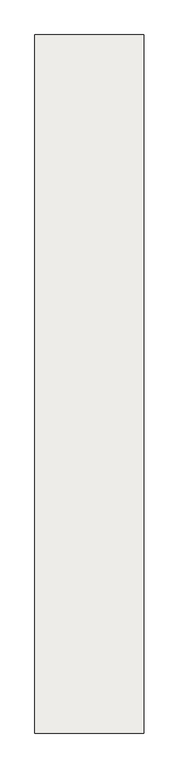
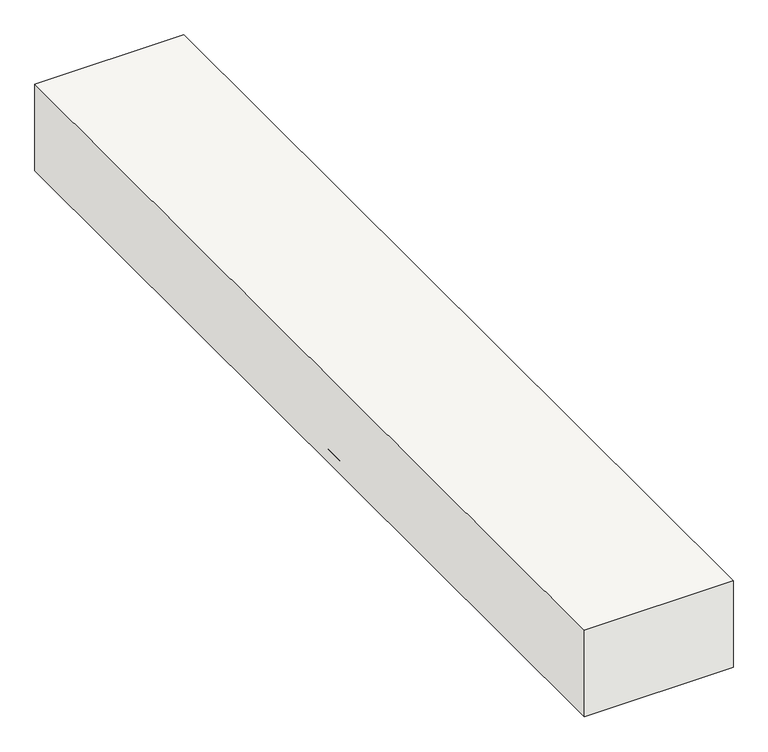
"""IFC4 building model written with IfcOpenShell, lengths in millimetres: slab geometry, Pano 16 (16 cm)."""

import ifcopenshell
import ifcopenshell.guid

model = None  # the IFC model being written
_history = None  # IfcOwnerHistory: only IFC2X3 demands one
_inside = {}  # id of a spatial element -> (the spatial element, [elements in it])
_under = {}  # id of a project, library or spatial element -> (it, [spatial elements below it])
_declared = {}  # id of a project -> (the project, [libraries it declares])
_typed = {}  # id of a type object -> (the type object, [elements of that type])
_made_of = {}  # id of a material, layer set ... -> (it, [elements and type objects made of it])


def new_model(schema):
    """Start an empty IFC model of exactly this schema.

    Asked for "IFC4X3", IfcOpenShell would pick the latest addendum, in which some entities
    have other attributes; the version numbers below select the first issue.
    IFC2X3 requires an IfcOwnerHistory on every rooted entity: one is made here for all.
    """
    global model, _history
    if schema == "IFC4X3":
        model = ifcopenshell.file(schema_version=(4, 3, 0, 0))
    else:
        model = ifcopenshell.file(schema=schema)
    _inside.clear()
    _under.clear()
    _declared.clear()
    _typed.clear()
    _made_of.clear()
    _history = None
    if model.schema == "IFC2X3":
        org = make("IfcOrganization", Name="unknown")
        user = make(
            "IfcPersonAndOrganization",
            ThePerson=make("IfcPerson", FamilyName="unknown"),
            TheOrganization=org,
        )
        app = make(
            "IfcApplication",
            ApplicationDeveloper=org,
            Version="unknown",
            ApplicationFullName="unknown",
            ApplicationIdentifier="unknown",
        )
        _history = make(
            "IfcOwnerHistory",
            OwningUser=user,
            OwningApplication=app,
            ChangeAction="ADDED",
            CreationDate=0,
        )
    return model


def make(cls, **values):
    """One entity of the class cls with the attributes given. An attribute that is None is left unset."""
    return model.create_entity(
        cls, **{name: value for name, value in values.items() if value is not None}
    )


def rooted(cls, **values):
    """An entity with a GlobalId (a new one), such as an element, a storey or a relation."""
    return make(cls, GlobalId=ifcopenshell.guid.new(), OwnerHistory=_history, **values)


def si_unit(unit_type, name, prefix=None):
    """IfcSIUnit, for example si_unit("LENGTHUNIT", "METRE", prefix="MILLI")."""
    return make("IfcSIUnit", UnitType=unit_type, Prefix=prefix, Name=name)


def assignment(units):
    """IfcUnitAssignment: the units of a project."""
    return None if units is None else make("IfcUnitAssignment", Units=units)


def point(xyz):
    """IfcCartesianPoint."""
    return None if xyz is None else make("IfcCartesianPoint", Coordinates=xyz)


def direction(xyz):
    """IfcDirection."""
    return None if xyz is None else make("IfcDirection", DirectionRatios=xyz)


def frame(location, z_axis=None, x_axis=None):
    """IfcAxis2Placement3D, a coordinate frame: its origin and axes. An axis left out is left unset."""
    return make(
        "IfcAxis2Placement3D",
        Location=point(location),
        Axis=direction(z_axis),
        RefDirection=direction(x_axis),
    )


def origin():
    """The frame at (0, 0, 0) with its axes left unset."""
    return frame((0.0, 0.0, 0.0))


def origin_with_axes():
    """The frame at (0, 0, 0) with the z axis (0, 0, 1) and the x axis (1, 0, 0) written out."""
    return frame((0.0, 0.0, 0.0), z_axis=(0.0, 0.0, 1.0), x_axis=(1.0, 0.0, 0.0))


def place(relative_to, where):
    """IfcLocalPlacement: puts the frame where relative to a parent placement (None: the world)."""
    return make(
        "IfcLocalPlacement", PlacementRelTo=relative_to, RelativePlacement=where
    )


def context(
    kind, dimensions, precision=None, world=None, true_north=None, identifier=None
):
    """IfcGeometricRepresentationContext, for example the 3D "Model" context."""
    return make(
        "IfcGeometricRepresentationContext",
        ContextIdentifier=identifier,
        ContextType=kind,
        CoordinateSpaceDimension=dimensions,
        Precision=precision,
        WorldCoordinateSystem=world,
        TrueNorth=true_north,
    )


def project(units=None, contexts=None):
    """IfcProject with its units and contexts."""
    return rooted(
        "IfcProject",
        Name="project",
        RepresentationContexts=contexts,
        UnitsInContext=assignment(units),
    )


def spatial(cls, under=None, at=None, **own):
    """A site, building, storey or space (cls), placed at a placement, below another one or the project."""
    s = rooted(cls, ObjectPlacement=at, **own)
    if under is not None:
        _under.setdefault(under.id(), (under, []))[1].append(s)
    return s


def polyline(points):
    """IfcPolyline through the points."""
    return make("IfcPolyline", Points=[point(p) for p in points])


def outline(outer, holes=None, kind="AREA"):
    """IfcArbitraryClosedProfileDef: a profile drawn as a closed curve; with holes, ...WithVoids."""
    if holes is None:
        return make("IfcArbitraryClosedProfileDef", ProfileType=kind, OuterCurve=outer)
    return make(
        "IfcArbitraryProfileDefWithVoids",
        ProfileType=kind,
        OuterCurve=outer,
        InnerCurves=holes,
    )


def extrude(swept, where, along, depth):
    """IfcExtrudedAreaSolid: the profile swept, set in the frame where, extruded along a direction by depth."""
    return make(
        "IfcExtrudedAreaSolid",
        SweptArea=swept,
        Position=where,
        ExtrudedDirection=direction(along),
        Depth=depth,
    )


def shape(context_of_items, identifier, shape_type, items):
    """IfcShapeRepresentation: the items that make up one representation, for example the "Body"."""
    return make(
        "IfcShapeRepresentation",
        ContextOfItems=context_of_items,
        RepresentationIdentifier=identifier,
        RepresentationType=shape_type,
        Items=items,
    )


def source(mapping_origin, context_of_items, identifier, shape_type, items):
    """IfcRepresentationMap: a shape defined once, which mapped items show again and again."""
    return make(
        "IfcRepresentationMap",
        MappingOrigin=mapping_origin,
        MappedRepresentation=shape(context_of_items, identifier, shape_type, items),
    )


def transform(
    local_origin,
    x_axis=None,
    y_axis=None,
    z_axis=None,
    scale=None,
    scale2=None,
    scale3=None,
    uniform=True,
):
    """IfcCartesianTransformationOperator3D, or its non-uniform kind. x_axis, y_axis, z_axis: its Axis1, 2, 3."""
    if uniform:
        return make(
            "IfcCartesianTransformationOperator3D",
            Axis1=direction(x_axis),
            Axis2=direction(y_axis),
            LocalOrigin=point(local_origin),
            Scale=scale,
            Axis3=direction(z_axis),
        )
    return make(
        "IfcCartesianTransformationOperator3DnonUniform",
        Axis1=direction(x_axis),
        Axis2=direction(y_axis),
        LocalOrigin=point(local_origin),
        Scale=scale,
        Axis3=direction(z_axis),
        Scale2=scale2,
        Scale3=scale3,
    )


def mapped(mapping_source, mapping_target):
    """IfcMappedItem: shows the shape of a source again, moved by a transform."""
    return make(
        "IfcMappedItem", MappingSource=mapping_source, MappingTarget=mapping_target
    )


def made_of(thing, what):
    """Note that an element or type object is made of a material, layer set ...; save() writes the relation."""
    if what is not None:
        _made_of.setdefault(what.id(), (what, []))[1].append(thing)
    return thing


def element(
    cls,
    number,
    at=None,
    inside=None,
    cuts=None,
    type_object=None,
    material=None,
    context=None,
    identifier="Body",
    shape_type=None,
    held_by="IfcProductDefinitionShape",
    body=None,
    shapes=None,
    **own,
):
    """One element of the class cls, such as IfcWall. Its Tag is "e" and its number.

    at: its placement. inside: the storey or other place that contains it. cuts: it is an
    opening in that element (IfcRelVoidsElement). A single representation is given by context,
    identifier, shape_type and body (its items); several are given by shapes. held_by: the class
    of the entity that holds the representations. save() writes the other relations.
    """
    e = rooted(cls, Tag="e%d" % number, ObjectPlacement=at, **own)
    if body is not None:
        shapes = [shape(context, identifier, shape_type, body)]
    if shapes is not None:
        e.Representation = make(held_by, Representations=shapes)
    if inside is not None:
        _inside.setdefault(inside.id(), (inside, []))[1].append(e)
    if cuts is not None:
        rooted(
            "IfcRelVoidsElement", RelatingBuildingElement=cuts, RelatedOpeningElement=e
        )
    if type_object is not None:
        _typed.setdefault(type_object.id(), (type_object, []))[1].append(e)
    return made_of(e, material)


def aggregate(whole, parts):
    """IfcRelAggregates: a whole, such as a stair, and the parts it consists of."""
    return rooted("IfcRelAggregates", RelatingObject=whole, RelatedObjects=parts)


def save(model, path):
    """Write the relations noted so far, then the file.

    IfcRelAggregates (storeys below a building ...), IfcRelContainedInSpatialStructure (elements
    in a storey), IfcRelDefinesByType, IfcRelAssociatesMaterial and IfcRelDeclares: one each for
    every whole, place, type object, material and project.
    """
    for whole, parts in _under.values():
        aggregate(whole, parts)
    for where, things in _inside.values():
        rooted(
            "IfcRelContainedInSpatialStructure",
            RelatedElements=things,
            RelatingStructure=where,
        )
    for kind, things in _typed.values():
        rooted("IfcRelDefinesByType", RelatedObjects=things, RelatingType=kind)
    for what, things in _made_of.values():
        rooted("IfcRelAssociatesMaterial", RelatedObjects=things, RelatingMaterial=what)
    for by, libraries in _declared.values():
        rooted("IfcRelDeclares", RelatingContext=by, RelatedDefinitions=libraries)
    model.write(path)


def slab_299a6d98(model_context):
    return source(origin(), model_context, "Body", "SweptSolid", [
        extrude(outline(polyline([(9400.0, 5350.0), (9660.0, 5350.0), (9660.0, 3685.0), (9400.0, 3685.0), (9400.0, 5350.0)])), origin_with_axes(), (0.0, 0.0, 1.0), 160.0),
        extrude(outline(polyline([(9400.0, 4855.0), (9400.0, 4995.0), (9660.0, 4995.0), (9660.0, 4855.0), (9400.0, 4855.0)])), origin_with_axes(), (0.0, 0.0, 1.0), 24.0),
        extrude(outline(polyline([(9400.0, 3855.0), (9400.0, 3995.0), (9660.0, 3995.0), (9660.0, 3855.0), (9400.0, 3855.0)])), origin_with_axes(), (0.0, 0.0, 1.0), 24.0),
        extrude(outline(polyline([(9400.0, 4355.0), (9400.0, 4495.0), (9660.0, 4495.0), (9660.0, 4355.0), (9400.0, 4355.0)])), origin_with_axes(), (0.0, 0.0, 1.0), 24.0),
    ])


if __name__ == "__main__":
    model = new_model("IFC4")
    model_context = context("Model", 3, world=origin())
    ifc_project = project(units=[si_unit("LENGTHUNIT", "METRE", prefix="MILLI")], contexts=[model_context])
    site = spatial("IfcSite", under=ifc_project)
    building = spatial("IfcBuilding", under=site)
    placement = place(None, origin())
    slab_shape = slab_299a6d98(model_context)
    element("IfcSlab", 1, ObjectType="Pano 16 (16 cm)", at=placement, inside=building, context=model_context, shape_type="MappedRepresentation", body=[
        mapped(slab_shape, transform((0.0, 0.0, 0.0), x_axis=(1.0, 0.0, 0.0), y_axis=(0.0, 1.0, 0.0), z_axis=(0.0, 0.0, 1.0))),
    ])
    save(model, "model.ifc")

# Revit data of these elements
# Element 1 (IfcSlab, "Pano 16 (16 cm)")
#   Materials on its faces: "Concreto armado", "RGB 168-169-158"
# Materials
#   "Concreto armado": class "Não atribuído", colour RGB 168 169 158, transparency 0
#   "RGB 168-169-158": class "Não atribuído", colour RGB 168 169 158, transparency 0
